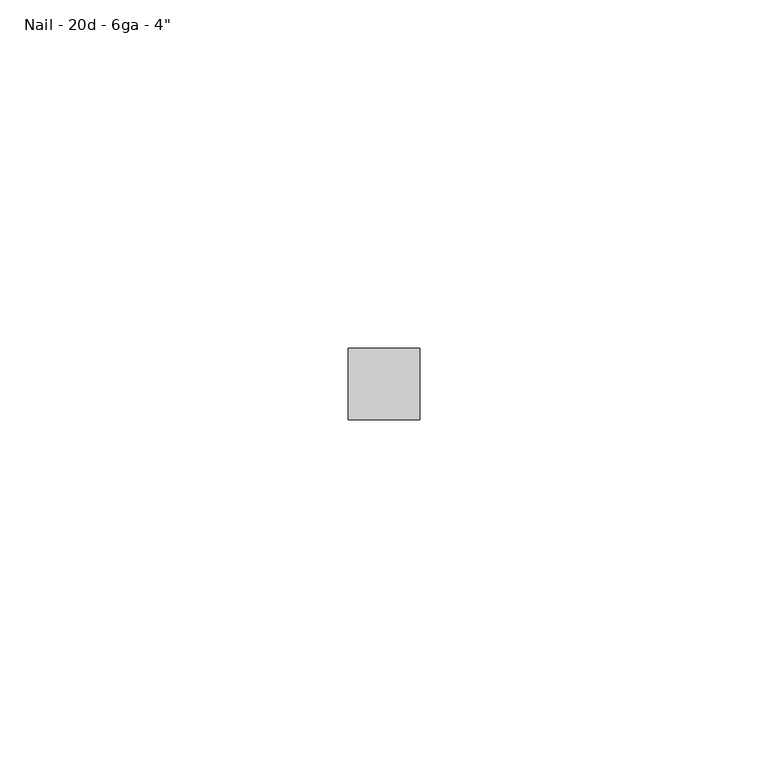
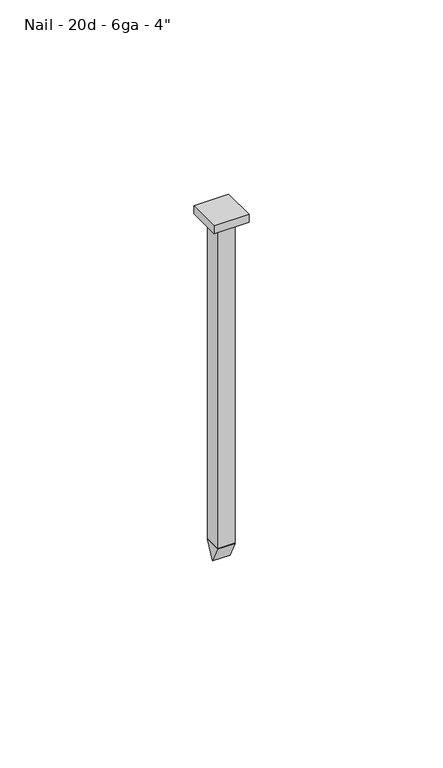
"""IFC4 building model written with IfcOpenShell, lengths in millimetres: fastener geometry."""

from ifc_helpers import new_model, si_unit, frame, origin, origin_with_axes, place, context, project, spatial, polyline, outline, extrude, source, transform, mapped, element, save


def fastener_57aff0e7(model_context):
    return source(origin(), model_context, "Body", "SweptSolid", [
        extrude(outline(polyline([(0.0, -106.7562), (-2.5781, -101.6), (2.5781, -101.6), (0.0, -106.7562)])), frame((-2.5781, 0.0, 0.0), z_axis=(1.0, 0.0, 0.0), x_axis=(0.0, 1.0, 0.0)), (0.0, 0.0, 1.0), 5.1562),
        extrude(outline(polyline([(-5.1562, -5.1562), (-5.1562, 5.1562), (5.1562, 5.1562), (5.1562, -5.1562), (-5.1562, -5.1562)])), origin_with_axes(), (0.0, 0.0, 1.0), 2.5781),
        extrude(outline(polyline([(-2.5781, 2.5781), (2.5781, 2.5781), (2.5781, -2.5781), (-2.5781, -2.5781), (-2.5781, 2.5781)])), frame((0.0, 0.0, -101.6), z_axis=(0.0, 0.0, 1.0), x_axis=(1.0, 0.0, 0.0)), (0.0, 0.0, 1.0), 101.6),
    ])


if __name__ == "__main__":
    model = new_model("IFC4")
    model_context = context("Model", 3, world=origin())
    ifc_project = project(units=[si_unit("LENGTHUNIT", "METRE", prefix="MILLI")], contexts=[model_context])
    site = spatial("IfcSite", under=ifc_project)
    building = spatial("IfcBuilding", under=site)
    placement = place(None, origin())
    fastener_shape = fastener_57aff0e7(model_context)
    element("IfcFastener", 1, ObjectType="060523 - W_P_C - Fastenings - Generic - SQUARE : Nail - 20d - 6ga - 4\"", at=placement, inside=building, context=model_context, shape_type="MappedRepresentation", body=[
        mapped(fastener_shape, transform((0.0, 0.0, 0.0), x_axis=(1.0, 0.0, 0.0), y_axis=(0.0, 1.0, 0.0), z_axis=(0.0, 0.0, 1.0))),
    ])
    save(model, "model.ifc")

# Revit data of these elements
# Type "060523 - W_P_C - Fastenings - Generic - SQUARE : Nail - 20d - 6ga - 4\""
#   Washer_Thickness = 0' - 0.00333"
#   Washer Radius = 0' - 0.1115"
#   Washer Offset - Head = 0' - 0"
#   Washer Offset = 0' - 0"
#   Thickness_of_Substrate [instance default] = 0' - 1"
#   Side = 0' - 0 37/64"
#   Radius = 0' - 0.1015"
#   Length [instance default] = 0' - 4"
#   Head Size = 0' - 1"
#   Head Radius = 0' - 0 1/2"
#   Head Height = 0' - 0.01"
#   Double Diameter = 0' - 0.406"
#   Diameter = 0' - 0.203"
#   Default Elevation = 4' - 0"
#   Washer_Nut_Visibility = no
#   Washer_Head_Visibility = no
#   Round_Head_Visibility = yes
#   Point Visibility = yes
#   Nut_Visibility = no
#   Hex_Head_Visiblilty = no
#   Washer Material = none
#   Bolt Material (Size) = AT SILL - FASTENER AT 24" O.C.
# Materials
#   "AT SILL - FASTENER AT 24\" O.C.": class "Generic", colour RGB 120 120 120, transparency 0, Cost = 0
